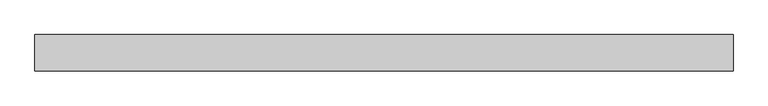
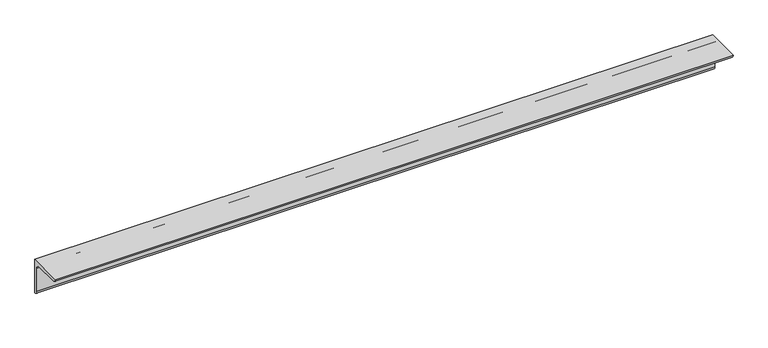
"""IFC4 building model written with IfcOpenShell, lengths in millimetres: beam geometry, 0912_Steel Framing_L-KSD3502 : H_SB_AR_S04_L-100x100x10_KBR2."""

from ifc_helpers import new_model, si_unit, point, frame, frame_2d, origin, place, context, project, spatial, polyline, circle_curve, trimmed, segment, composite_curve, outline, extrude, source, transform, mapped, element, save


def beam_df177b35(model_context):
    return source(origin(), model_context, "Body", "SweptSolid", [
        extrude(outline(composite_curve([segment(polyline([(28.2, 28.2), (28.2, -71.8)]), True, "CONTINUOUS"), segment(trimmed(circle_curve(frame_2d((28.2, -61.8)), 10.0), [point((28.2, -71.8))], [point((18.2, -61.8))], False, "CARTESIAN"), True, "CONTINUOUS"), segment(polyline([(18.2, -61.8), (18.2, 8.2)]), True, "CONTINUOUS"), segment(trimmed(circle_curve(frame_2d((8.2, 8.2)), 10.0), [point((18.2, 8.2))], [point((8.2, 18.2))], True, "CARTESIAN"), True, "CONTINUOUS"), segment(polyline([(8.2, 18.2), (-61.8, 18.2)]), True, "CONTINUOUS"), segment(trimmed(circle_curve(frame_2d((-61.8, 28.2)), 10.0), [point((-61.8, 18.2))], [point((-71.8, 28.2))], False, "CARTESIAN"), True, "CONTINUOUS"), segment(polyline([(-71.8, 28.2), (28.2, 28.2)]), True, "CONTINUOUS")], self_intersect=False)), frame((-947.4772619, 0.0, 0.0), z_axis=(1.0, 0.0, 0.0), x_axis=(0.0, 1.0, 0.0)), (0.0, 0.0, 1.0), 1921.8464173),
    ])


if __name__ == "__main__":
    model = new_model("IFC4")
    model_context = context("Model", 3, world=origin())
    ifc_project = project(units=[si_unit("LENGTHUNIT", "METRE", prefix="MILLI")], contexts=[model_context])
    site = spatial("IfcSite", under=ifc_project)
    building = spatial("IfcBuilding", under=site)
    placement = place(None, origin())
    beam_shape = beam_df177b35(model_context)
    element("IfcBeam", 1, ObjectType="0912_Steel Framing_L-KSD3502 : H_SB_AR_S04_L-100x100x10_KBR2", at=placement, inside=building, context=model_context, shape_type="MappedRepresentation", body=[
        mapped(beam_shape, transform((0.0, 0.0, 0.0), x_axis=(1.0, 0.0, 0.0), y_axis=(0.0, 1.0, 0.0), z_axis=(0.0, 0.0, 1.0))),
    ])
    save(model, "model.ifc")

# Revit data of these elements
# Type "0912_Steel Framing_L-KSD3502 : H_SB_AR_S04_L-100x100x10_KBR2"
#   k = 25 mm
#   Perimeter = 0.40 m²/m
#   Nominal Weight = 14.90 kgf/m
#   Length [instance default] = 1000 mm
#   b = 100 mm
#   d = 100 mm
#   t = 10 mm
#   x = 28.2 mm
#   y = 28.2 mm
#   A = 1900.00 m²
#   Structural Material [instance default] = Steel, 45-345
# Element 1 (IfcBeam, "0912_Steel Framing_L-KSD3502 : H_SB_AR_S04_L-100x100x10_KBR2")
#   Structural Material = Steel ASTM A36
#   Materials on its faces: "Steel ASTM A36"
# Materials
#   "Steel, 45-345": class "Metal", colour RGB 189 187 185, transparency 0, Description = "Steel 345 MPa", Cost = 0
#   "Steel ASTM A36": class "Metal", colour RGB 199 199 199, transparency 0, Description = "Structural steel, ASTM A36 Grade B, mill finish", Cost = 0
